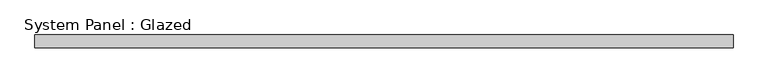
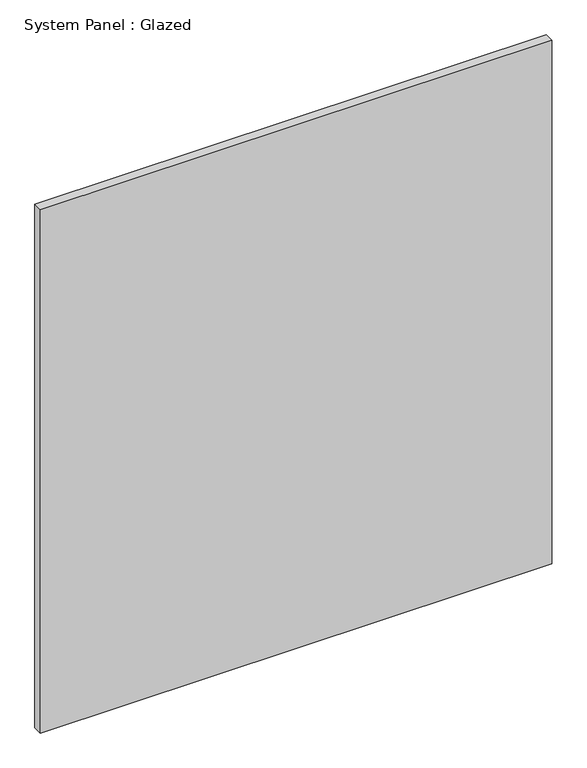
"""IFC4 building model written with IfcOpenShell, lengths in millimetres: plate geometry, System Panel : Glazed."""

from ifc_helpers import new_model, si_unit, origin, origin_with_axes, place, context, project, spatial, polyline, outline, extrude, source, transform, mapped, element, save


def system_panel_glazed_fe22fd77(model_context):
    return source(origin(), model_context, "Body", "SweptSolid", [
        extrude(outline(polyline([(682.4999999, 24.5), (-682.4999999, 24.5), (-682.4999999, 49.5), (682.4999999, 49.5), (682.4999999, 24.5)])), origin_with_axes(), (0.0, 0.0, 1.0), 1476.6044889),
    ])


if __name__ == "__main__":
    model = new_model("IFC4")
    model_context = context("Model", 3, world=origin())
    ifc_project = project(units=[si_unit("LENGTHUNIT", "METRE", prefix="MILLI")], contexts=[model_context])
    site = spatial("IfcSite", under=ifc_project)
    building = spatial("IfcBuilding", under=site)
    placement = place(None, origin())
    system_panel_glazed_shape = system_panel_glazed_fe22fd77(model_context)
    element("IfcPlate", 1, ObjectType="System Panel : Glazed", at=placement, inside=building, context=model_context, shape_type="MappedRepresentation", body=[
        mapped(system_panel_glazed_shape, transform((0.0, 0.0, 0.0), x_axis=(1.0, 0.0, 0.0), y_axis=(0.0, 1.0, 0.0), z_axis=(0.0, 0.0, 1.0))),
    ])
    save(model, "model.ifc")

# Revit data of these elements
# Element 1 (IfcPlate, "System Panel : Glazed")
#   Materials on its faces: "Glass"
# Materials
#   "Glass": class "Glass", colour RGB 218 227 224, transparency 0.85, Description = "Soda Lime Glass", Cost = 0
